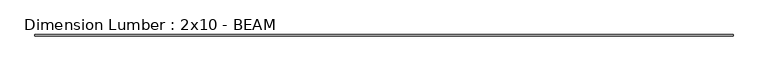
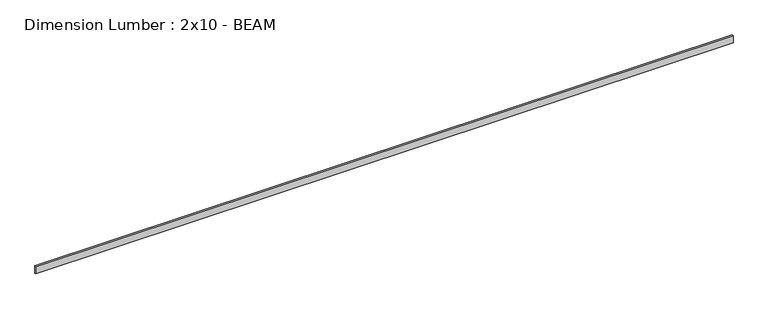
"""IFC4 building model written with IfcOpenShell, lengths in millimetres: beam geometry, Dimension Lumber : 2x10 - BEAM."""

from ifc_helpers import new_model, si_unit, frame, origin, place, context, project, spatial, polyline, outline, extrude, source, transform, mapped, element, save


def dimension_lumber_2x10_beam_6c8e5ac9(model_context):
    return source(origin(), model_context, "Body", "SweptSolid", [
        extrude(outline(polyline([(10510.04375, 19.05), (10510.04375, -19.05), (-10768.80625, -19.05), (-10768.80625, 19.05), (10510.04375, 19.05)])), frame((0.0, 0.0, -117.475), z_axis=(0.0, 0.0, 1.0), x_axis=(1.0, 0.0, 0.0)), (0.0, 0.0, 1.0), 234.95),
    ])


if __name__ == "__main__":
    model = new_model("IFC4")
    model_context = context("Model", 3, world=origin())
    ifc_project = project(units=[si_unit("LENGTHUNIT", "METRE", prefix="MILLI")], contexts=[model_context])
    site = spatial("IfcSite", under=ifc_project)
    building = spatial("IfcBuilding", under=site)
    placement = place(None, origin())
    dimension_lumber_2x10_beam_shape = dimension_lumber_2x10_beam_6c8e5ac9(model_context)
    element("IfcBeam", 1, ObjectType="Dimension Lumber : 2x10 - BEAM", at=placement, inside=building, context=model_context, shape_type="MappedRepresentation", body=[
        mapped(dimension_lumber_2x10_beam_shape, transform((0.0, 0.0, 0.0), x_axis=(1.0, 0.0, 0.0), y_axis=(0.0, 1.0, 0.0), z_axis=(0.0, 0.0, 1.0))),
    ])
    save(model, "model.ifc")

# Revit data of these elements
# Type "Dimension Lumber : 2x10 - BEAM"
#   Assembly Code = "B10"
#   A = 0.0755556 SF
#   Length [instance default] = 5' - 0"
#   b = 0' - 1 1/2"
#   d = 0' - 9 1/4"
#   Structural Material = (3) SISTERED 2X10s AT BEAM
# Element 1 (IfcBeam, "Dimension Lumber : 2x10 - BEAM")
#   Materials on its faces: "(3) SISTERED 2X10s AT BEAM"
# Materials
#   "(3) SISTERED 2X10s AT BEAM": class "Wood", colour RGB 234 198 147, transparency 0, Description = "Pinus Echinata", Cost = 0
